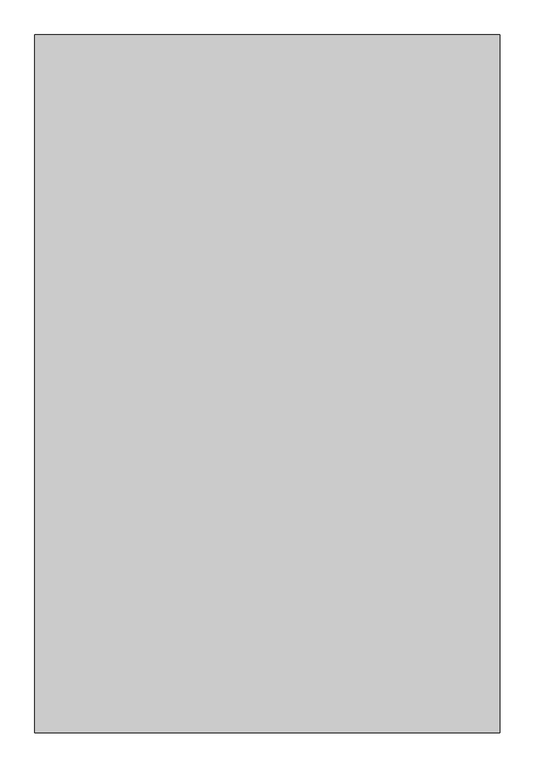
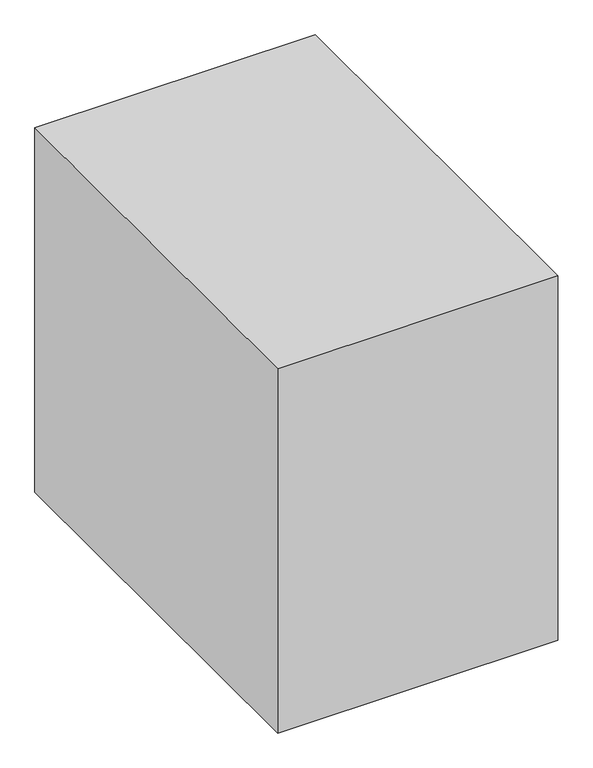
"""IFC4 building model written with IfcOpenShell, lengths in millimetres: proxy geometry, Space Planning Box_hec : Space Planning Box_hec."""

import ifcopenshell
import ifcopenshell.guid

model = None  # the IFC model being written
_history = None  # IfcOwnerHistory: only IFC2X3 demands one
_inside = {}  # id of a spatial element -> (the spatial element, [elements in it])
_under = {}  # id of a project, library or spatial element -> (it, [spatial elements below it])
_declared = {}  # id of a project -> (the project, [libraries it declares])
_typed = {}  # id of a type object -> (the type object, [elements of that type])
_made_of = {}  # id of a material, layer set ... -> (it, [elements and type objects made of it])


def new_model(schema):
    """Start an empty IFC model of exactly this schema.

    Asked for "IFC4X3", IfcOpenShell would pick the latest addendum, in which some entities
    have other attributes; the version numbers below select the first issue.
    IFC2X3 requires an IfcOwnerHistory on every rooted entity: one is made here for all.
    """
    global model, _history
    if schema == "IFC4X3":
        model = ifcopenshell.file(schema_version=(4, 3, 0, 0))
    else:
        model = ifcopenshell.file(schema=schema)
    _inside.clear()
    _under.clear()
    _declared.clear()
    _typed.clear()
    _made_of.clear()
    _history = None
    if model.schema == "IFC2X3":
        org = make("IfcOrganization", Name="unknown")
        user = make(
            "IfcPersonAndOrganization",
            ThePerson=make("IfcPerson", FamilyName="unknown"),
            TheOrganization=org,
        )
        app = make(
            "IfcApplication",
            ApplicationDeveloper=org,
            Version="unknown",
            ApplicationFullName="unknown",
            ApplicationIdentifier="unknown",
        )
        _history = make(
            "IfcOwnerHistory",
            OwningUser=user,
            OwningApplication=app,
            ChangeAction="ADDED",
            CreationDate=0,
        )
    return model


def make(cls, **values):
    """One entity of the class cls with the attributes given. An attribute that is None is left unset."""
    return model.create_entity(
        cls, **{name: value for name, value in values.items() if value is not None}
    )


def rooted(cls, **values):
    """An entity with a GlobalId (a new one), such as an element, a storey or a relation."""
    return make(cls, GlobalId=ifcopenshell.guid.new(), OwnerHistory=_history, **values)


def si_unit(unit_type, name, prefix=None):
    """IfcSIUnit, for example si_unit("LENGTHUNIT", "METRE", prefix="MILLI")."""
    return make("IfcSIUnit", UnitType=unit_type, Prefix=prefix, Name=name)


def assignment(units):
    """IfcUnitAssignment: the units of a project."""
    return None if units is None else make("IfcUnitAssignment", Units=units)


def point(xyz):
    """IfcCartesianPoint."""
    return None if xyz is None else make("IfcCartesianPoint", Coordinates=xyz)


def direction(xyz):
    """IfcDirection."""
    return None if xyz is None else make("IfcDirection", DirectionRatios=xyz)


def frame(location, z_axis=None, x_axis=None):
    """IfcAxis2Placement3D, a coordinate frame: its origin and axes. An axis left out is left unset."""
    return make(
        "IfcAxis2Placement3D",
        Location=point(location),
        Axis=direction(z_axis),
        RefDirection=direction(x_axis),
    )


def origin():
    """The frame at (0, 0, 0) with its axes left unset."""
    return frame((0.0, 0.0, 0.0))


def origin_with_axes():
    """The frame at (0, 0, 0) with the z axis (0, 0, 1) and the x axis (1, 0, 0) written out."""
    return frame((0.0, 0.0, 0.0), z_axis=(0.0, 0.0, 1.0), x_axis=(1.0, 0.0, 0.0))


def place(relative_to, where):
    """IfcLocalPlacement: puts the frame where relative to a parent placement (None: the world)."""
    return make(
        "IfcLocalPlacement", PlacementRelTo=relative_to, RelativePlacement=where
    )


def context(
    kind, dimensions, precision=None, world=None, true_north=None, identifier=None
):
    """IfcGeometricRepresentationContext, for example the 3D "Model" context."""
    return make(
        "IfcGeometricRepresentationContext",
        ContextIdentifier=identifier,
        ContextType=kind,
        CoordinateSpaceDimension=dimensions,
        Precision=precision,
        WorldCoordinateSystem=world,
        TrueNorth=true_north,
    )


def project(units=None, contexts=None):
    """IfcProject with its units and contexts."""
    return rooted(
        "IfcProject",
        Name="project",
        RepresentationContexts=contexts,
        UnitsInContext=assignment(units),
    )


def spatial(cls, under=None, at=None, **own):
    """A site, building, storey or space (cls), placed at a placement, below another one or the project."""
    s = rooted(cls, ObjectPlacement=at, **own)
    if under is not None:
        _under.setdefault(under.id(), (under, []))[1].append(s)
    return s


def polyline(points):
    """IfcPolyline through the points."""
    return make("IfcPolyline", Points=[point(p) for p in points])


def outline(outer, holes=None, kind="AREA"):
    """IfcArbitraryClosedProfileDef: a profile drawn as a closed curve; with holes, ...WithVoids."""
    if holes is None:
        return make("IfcArbitraryClosedProfileDef", ProfileType=kind, OuterCurve=outer)
    return make(
        "IfcArbitraryProfileDefWithVoids",
        ProfileType=kind,
        OuterCurve=outer,
        InnerCurves=holes,
    )


def extrude(swept, where, along, depth):
    """IfcExtrudedAreaSolid: the profile swept, set in the frame where, extruded along a direction by depth."""
    return make(
        "IfcExtrudedAreaSolid",
        SweptArea=swept,
        Position=where,
        ExtrudedDirection=direction(along),
        Depth=depth,
    )


def shape(context_of_items, identifier, shape_type, items):
    """IfcShapeRepresentation: the items that make up one representation, for example the "Body"."""
    return make(
        "IfcShapeRepresentation",
        ContextOfItems=context_of_items,
        RepresentationIdentifier=identifier,
        RepresentationType=shape_type,
        Items=items,
    )


def source(mapping_origin, context_of_items, identifier, shape_type, items):
    """IfcRepresentationMap: a shape defined once, which mapped items show again and again."""
    return make(
        "IfcRepresentationMap",
        MappingOrigin=mapping_origin,
        MappedRepresentation=shape(context_of_items, identifier, shape_type, items),
    )


def transform(
    local_origin,
    x_axis=None,
    y_axis=None,
    z_axis=None,
    scale=None,
    scale2=None,
    scale3=None,
    uniform=True,
):
    """IfcCartesianTransformationOperator3D, or its non-uniform kind. x_axis, y_axis, z_axis: its Axis1, 2, 3."""
    if uniform:
        return make(
            "IfcCartesianTransformationOperator3D",
            Axis1=direction(x_axis),
            Axis2=direction(y_axis),
            LocalOrigin=point(local_origin),
            Scale=scale,
            Axis3=direction(z_axis),
        )
    return make(
        "IfcCartesianTransformationOperator3DnonUniform",
        Axis1=direction(x_axis),
        Axis2=direction(y_axis),
        LocalOrigin=point(local_origin),
        Scale=scale,
        Axis3=direction(z_axis),
        Scale2=scale2,
        Scale3=scale3,
    )


def mapped(mapping_source, mapping_target):
    """IfcMappedItem: shows the shape of a source again, moved by a transform."""
    return make(
        "IfcMappedItem", MappingSource=mapping_source, MappingTarget=mapping_target
    )


def made_of(thing, what):
    """Note that an element or type object is made of a material, layer set ...; save() writes the relation."""
    if what is not None:
        _made_of.setdefault(what.id(), (what, []))[1].append(thing)
    return thing


def element(
    cls,
    number,
    at=None,
    inside=None,
    cuts=None,
    type_object=None,
    material=None,
    context=None,
    identifier="Body",
    shape_type=None,
    held_by="IfcProductDefinitionShape",
    body=None,
    shapes=None,
    **own,
):
    """One element of the class cls, such as IfcWall. Its Tag is "e" and its number.

    at: its placement. inside: the storey or other place that contains it. cuts: it is an
    opening in that element (IfcRelVoidsElement). A single representation is given by context,
    identifier, shape_type and body (its items); several are given by shapes. held_by: the class
    of the entity that holds the representations. save() writes the other relations.
    """
    e = rooted(cls, Tag="e%d" % number, ObjectPlacement=at, **own)
    if body is not None:
        shapes = [shape(context, identifier, shape_type, body)]
    if shapes is not None:
        e.Representation = make(held_by, Representations=shapes)
    if inside is not None:
        _inside.setdefault(inside.id(), (inside, []))[1].append(e)
    if cuts is not None:
        rooted(
            "IfcRelVoidsElement", RelatingBuildingElement=cuts, RelatedOpeningElement=e
        )
    if type_object is not None:
        _typed.setdefault(type_object.id(), (type_object, []))[1].append(e)
    return made_of(e, material)


def aggregate(whole, parts):
    """IfcRelAggregates: a whole, such as a stair, and the parts it consists of."""
    return rooted("IfcRelAggregates", RelatingObject=whole, RelatedObjects=parts)


def save(model, path):
    """Write the relations noted so far, then the file.

    IfcRelAggregates (storeys below a building ...), IfcRelContainedInSpatialStructure (elements
    in a storey), IfcRelDefinesByType, IfcRelAssociatesMaterial and IfcRelDeclares: one each for
    every whole, place, type object, material and project.
    """
    for whole, parts in _under.values():
        aggregate(whole, parts)
    for where, things in _inside.values():
        rooted(
            "IfcRelContainedInSpatialStructure",
            RelatedElements=things,
            RelatingStructure=where,
        )
    for kind, things in _typed.values():
        rooted("IfcRelDefinesByType", RelatedObjects=things, RelatingType=kind)
    for what, things in _made_of.values():
        rooted("IfcRelAssociatesMaterial", RelatedObjects=things, RelatingMaterial=what)
    for by, libraries in _declared.values():
        rooted("IfcRelDeclares", RelatingContext=by, RelatedDefinitions=libraries)
    model.write(path)


def generic_models_cc1dae17(model_context):
    return source(origin(), model_context, "Body", "SweptSolid", [
        extrude(outline(polyline([(2000.0, 3000.0), (2000.0, -3000.0), (-2000.0, -3000.0), (-2000.0, 3000.0), (2000.0, 3000.0)])), origin_with_axes(), (0.0, 0.0, 1.0), 5500.0),
    ])


if __name__ == "__main__":
    model = new_model("IFC4")
    model_context = context("Model", 3, world=origin())
    ifc_project = project(units=[si_unit("LENGTHUNIT", "METRE", prefix="MILLI")], contexts=[model_context])
    site = spatial("IfcSite", under=ifc_project)
    building = spatial("IfcBuilding", under=site)
    placement = place(None, origin())
    generic_models_shape = generic_models_cc1dae17(model_context)
    element("IfcBuildingElementProxy", 1, Name="Space Planning Box_hec : Space Planning Box_hec", ObjectType="Space Planning Box_hec : Space Planning Box_hec", at=placement, inside=building, context=model_context, shape_type="MappedRepresentation", body=[
        mapped(generic_models_shape, transform((0.0, 0.0, 0.0), x_axis=(1.0, 0.0, 0.0), y_axis=(0.0, 1.0, 0.0), z_axis=(0.0, 0.0, 1.0))),
    ])
    save(model, "model.ifc")

# Revit data of these elements
# Type "Space Planning Box_hec : Space Planning Box_hec"
#   Type Comments = "..."
#   Room Name [instance default] = "?"
#   Interior Finish [instance default] = ""
#   Exterior Finish [instance default] = ""
#   Department [instance default] = ""
#   Assembly Code = "..."
#   ceiling height [instance default] = 0
#   Width [instance default] = 1524 mm
#   Program Area [instance default] = 0.00 m²
#   Length [instance default] = 1524 mm
#   Height [instance default] = 1524 mm
#   Area [instance default] = 2.32258 m²
#   Fill Color [instance default] = Cyan
#   Default Elevation = 0
# Element 1 (IfcBuildingElementProxy, "Space Planning Box_hec : Space Planning Box_hec")
#   Room Name = "Staircase"
#   Exterior Finish = "N/A..N/A,,EW2..N/A..N/A"
#   Department = "PATHV1"
#   Width = 4000 mm
#   Program Area = 24.00 m²
#   Length = 6000 mm
#   Height = 5500 mm
#   Area = 24.00 m²
#   Fill Color = Green
#   Materials on its faces: "Green"
# Materials
#   "Cyan": class "Generic", colour RGB 0 255 255, transparency 0.2, Cost = 0
#   "Green": class "Generic", colour RGB 0 128 0, transparency 0.2, Cost = 0
